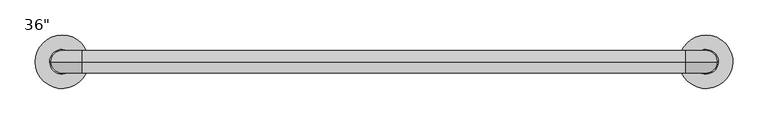
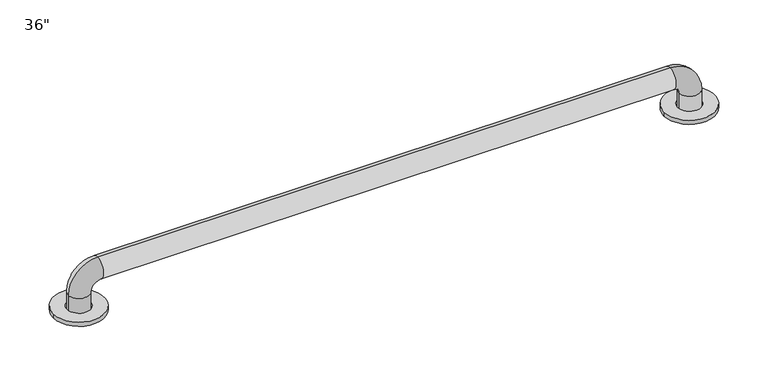
"""IFC4 building model written with IfcOpenShell, lengths in millimetres: proxy geometry."""

from ifc_helpers import new_model, si_unit, point, frame, frame_2d, origin, origin_with_axes, origin_2d, place, context, project, spatial, circle_curve, ellipse_curve, trimmed, segment, composite_curve, outline, extrude, source, transform, mapped, element, save
from ifc_brep_helpers import plane_surface, cylinder_surface, revolved_surface, advanced_brep


def proxy_c78fe107(model_context):
    return source(origin(), model_context, "Body", "SolidModel", [
        extrude(outline(composite_curve([segment(trimmed(circle_curve(frame_2d((914.4, 0.0)), 38.1), [point((876.3, 0.0))], [point((914.4, 38.1))], False, "CARTESIAN"), True, "CONTINUOUS"), segment(trimmed(circle_curve(frame_2d((914.4, 0.0)), 38.1), [point((914.4, 38.1))], [point((876.3, 0.0))], False, "CARTESIAN"), True, "CONTINUOUS")], self_intersect=False), holes=[composite_curve([segment(trimmed(circle_curve(frame_2d((914.4, 0.0)), 17.4625), [point((896.9375, 0.0))], [point((914.4, 17.4625))], True, "CARTESIAN"), True, "CONTINUOUS"), segment(trimmed(circle_curve(frame_2d((914.4, 0.0)), 17.4625), [point((914.4, 17.4625))], [point((896.9375, 0.0))], True, "CARTESIAN"), True, "CONTINUOUS")], self_intersect=False)]), origin_with_axes(), (0.0, 0.0, 1.0), 6.35),
        extrude(outline(composite_curve([segment(trimmed(circle_curve(origin_2d(), 38.1), [point((-38.1, 0.0))], [point((0.0, 38.1))], False, "CARTESIAN"), True, "CONTINUOUS"), segment(trimmed(circle_curve(origin_2d(), 38.1), [point((0.0, 38.1))], [point((-38.1, 0.0))], False, "CARTESIAN"), True, "CONTINUOUS")], self_intersect=False), holes=[composite_curve([segment(trimmed(circle_curve(origin_2d(), 17.4625), [point((-17.4625, 0.0))], [point((0.0, 17.4625))], True, "CARTESIAN"), True, "CONTINUOUS"), segment(trimmed(circle_curve(origin_2d(), 17.4625), [point((0.0, 17.4625))], [point((-17.4625, 0.0))], True, "CARTESIAN"), True, "CONTINUOUS")], self_intersect=False)]), origin_with_axes(), (0.0, 0.0, 1.0), 6.35),
        advanced_brep(
        [(930.275, 0.0, 0.0), (898.525, 0.0, 0.0), (898.525, 0.0, 28.575), (930.275, 0.0, 28.575), (885.825, 0.0, 41.275), (885.825, 0.0, 73.025), (28.575, 0.0, 41.275), (28.575, 0.0, 73.025), (15.875, 0.0, 28.575), (-15.875, 0.0, 28.575), (-15.875, 0.0, 0.0), (15.875, 0.0, 0.0)],
        [
            (0, 1, circle_curve(frame((914.4, 0.0, 0.0), z_axis=(0.0, 0.0, -1.0), x_axis=(-1.0, 0.0, 0.0)), 15.875)),
            (1, 0, circle_curve(frame((914.4, 0.0, 0.0), z_axis=(0.0, 0.0, -1.0), x_axis=(-1.0, 0.0, 0.0)), 15.875)),
            (1, 2),
            (2, 3, circle_curve(frame((914.4, 0.0, 28.575), z_axis=(0.0, 0.0, -1.0), x_axis=(-1.0, 0.0, 0.0)), 15.875)),
            (3, 0),
            (3, 2, circle_curve(frame((914.4, 0.0, 28.575), z_axis=(0.0, 0.0, -1.0), x_axis=(-1.0, 0.0, 0.0)), 15.875)),
            (4, 5, circle_curve(frame((885.825, 0.0, 57.15), z_axis=(1.0, 0.0, 0.0), x_axis=(0.0, 0.0, -1.0)), 15.875)),
            (5, 3, circle_curve(frame((885.825, 0.0, 28.575), z_axis=(0.0, 1.0, 0.0), x_axis=(1.0, 0.0, 0.0)), 44.45)),
            (2, 4, circle_curve(frame((885.825, 0.0, 28.575), z_axis=(0.0, -1.0, 0.0), x_axis=(1.0, 0.0, 0.0)), 12.7)),
            (5, 4, circle_curve(frame((885.825, 0.0, 57.15), z_axis=(1.0, 0.0, 0.0), x_axis=(0.0, 0.0, -1.0)), 15.875)),
            (4, 6),
            (6, 7, circle_curve(frame((28.575, 0.0, 57.15), z_axis=(1.0, 0.0, 0.0), x_axis=(0.0, 0.0, -1.0)), 15.875)),
            (7, 5),
            (7, 6, circle_curve(frame((28.575, 0.0, 57.15), z_axis=(1.0, 0.0, 0.0), x_axis=(0.0, 0.0, -1.0)), 15.875)),
            (8, 9, circle_curve(frame((0.0, 0.0, 28.575), z_axis=(0.0, 0.0, 1.0), x_axis=(1.0, 0.0, 0.0)), 15.875)),
            (9, 7, circle_curve(frame((28.575, 0.0, 28.575), z_axis=(0.0, 1.0, 0.0), x_axis=(0.0, 0.0, 1.0)), 44.45)),
            (6, 8, circle_curve(frame((28.575, 0.0, 28.575), z_axis=(0.0, -1.0, 0.0), x_axis=(0.0, 0.0, 1.0)), 12.7)),
            (9, 8, circle_curve(frame((0.0, 0.0, 28.575), z_axis=(0.0, 0.0, 1.0), x_axis=(1.0, 0.0, 0.0)), 15.875)),
            (10, 11, circle_curve(frame((0.0, 0.0, 0.0), z_axis=(0.0, 0.0, -1.0), x_axis=(1.0, 0.0, 0.0)), 15.875)),
            (11, 10, circle_curve(frame((0.0, 0.0, 0.0), z_axis=(0.0, 0.0, -1.0), x_axis=(1.0, 0.0, 0.0)), 15.875)),
            (8, 11),
            (10, 9),
        ],
        [
            plane_surface(frame((914.4, 0.0, 0.0), z_axis=(0.0, 0.0, -1.0), x_axis=(0.0, 1.0, 0.0))),
            cylinder_surface(frame((914.4, 0.0, 0.0), z_axis=(0.0, 0.0, -1.0), x_axis=(-1.0, 0.0, 0.0)), 15.875),
            revolved_surface(trimmed(ellipse_curve(frame((914.4, 0.0, 28.575), z_axis=(0.0, 0.0, 1.0), x_axis=(-1.0, 0.0, 0.0)), 15.875, 15.875), [point((930.275, 0.0, 28.575))], [point((898.525, 0.0, 28.575))], True, "CARTESIAN"), (885.825, 0.0, 28.575), (0.0, 1.0, 0.0)),
            revolved_surface(trimmed(ellipse_curve(frame((914.4, 0.0, 28.575), z_axis=(0.0, 0.0, 1.0), x_axis=(-1.0, 0.0, 0.0)), 15.875, 15.875), [point((898.525, 0.0, 28.575))], [point((930.275, 0.0, 28.575))], True, "CARTESIAN"), (885.825, 0.0, 28.575), (0.0, 1.0, 0.0)),
            cylinder_surface(frame((885.825, 0.0, 57.15), z_axis=(1.0, 0.0, 0.0), x_axis=(0.0, 0.0, -1.0)), 15.875),
            revolved_surface(trimmed(ellipse_curve(frame((28.575, 0.0, 57.15), z_axis=(-1.0, 0.0, 0.0), x_axis=(0.0, 0.0, -1.0)), 15.875, 15.875), [point((28.575, 0.0, 73.025))], [point((28.575, 0.0, 41.275))], True, "CARTESIAN"), (28.575, 0.0, 28.575), (0.0, 1.0, 0.0)),
            revolved_surface(trimmed(ellipse_curve(frame((28.575, 0.0, 57.15), z_axis=(-1.0, 0.0, 0.0), x_axis=(0.0, 0.0, -1.0)), 15.875, 15.875), [point((28.575, 0.0, 41.275))], [point((28.575, 0.0, 73.025))], True, "CARTESIAN"), (28.575, 0.0, 28.575), (0.0, 1.0, 0.0)),
            plane_surface(frame((0.0, 0.0, 0.0), z_axis=(0.0, 0.0, -1.0), x_axis=(0.0, 1.0, 0.0))),
            cylinder_surface(frame((0.0, 0.0, 28.575), z_axis=(0.0, 0.0, 1.0), x_axis=(1.0, 0.0, 0.0)), 15.875),
        ],
        [
            (0, [[1, 2]]),
            (1, [[3, 4, 5, -2]]),
            (1, [[-5, 6, -3, -1]]),
            (2, [[7, 8, -4, 9]]),
            (3, [[10, -9, -6, -8]]),
            (4, [[11, 12, 13, -7]]),
            (4, [[-13, 14, -11, -10]]),
            (5, [[15, 16, -12, 17]]),
            (6, [[18, -17, -14, -16]]),
            (7, [[19, 20]]),
            (8, [[21, -19, 22, -15]]),
            (8, [[-22, -20, -21, -18]]),
        ],
    ),
    ])


if __name__ == "__main__":
    model = new_model("IFC4")
    model_context = context("Model", 3, world=origin())
    ifc_project = project(units=[si_unit("LENGTHUNIT", "METRE", prefix="MILLI")], contexts=[model_context])
    site = spatial("IfcSite", under=ifc_project)
    building = spatial("IfcBuilding", under=site)
    placement = place(None, origin())
    proxy_shape = proxy_c78fe107(model_context)
    element("IfcBuildingElementProxy", 1, Name="Seqm-Grab Bar : 36\"", ObjectType="Seqm-Grab Bar : 36\"", at=placement, inside=building, context=model_context, shape_type="MappedRepresentation", body=[
        mapped(proxy_shape, transform((0.0, 0.0, 0.0), x_axis=(1.0, 0.0, 0.0), y_axis=(0.0, 1.0, 0.0), z_axis=(0.0, 0.0, 1.0))),
    ])
    save(model, "model.ifc")

# Revit data of these elements
# Type "Seqm-Grab Bar : 36\""
#   Spec Number = "10 28 00"
#   Spec Description = "36\" GRAB BAR"
#   Length = 3' - 0"
#   Default Elevation = 4' - 0"
#   Grab Bar Material = GRAB BARS - AT ADA RESTROOMS ONLY
# Element 1 (IfcBuildingElementProxy, "Seqm-Grab Bar : 36\"")
#   Materials on its faces: "GRAB BARS - AT ADA RESTROOMS ONLY"
# Materials
#   "GRAB BARS - AT ADA RESTROOMS ONLY": class "Generic", colour RGB 120 120 120, transparency 0, Cost = 0
